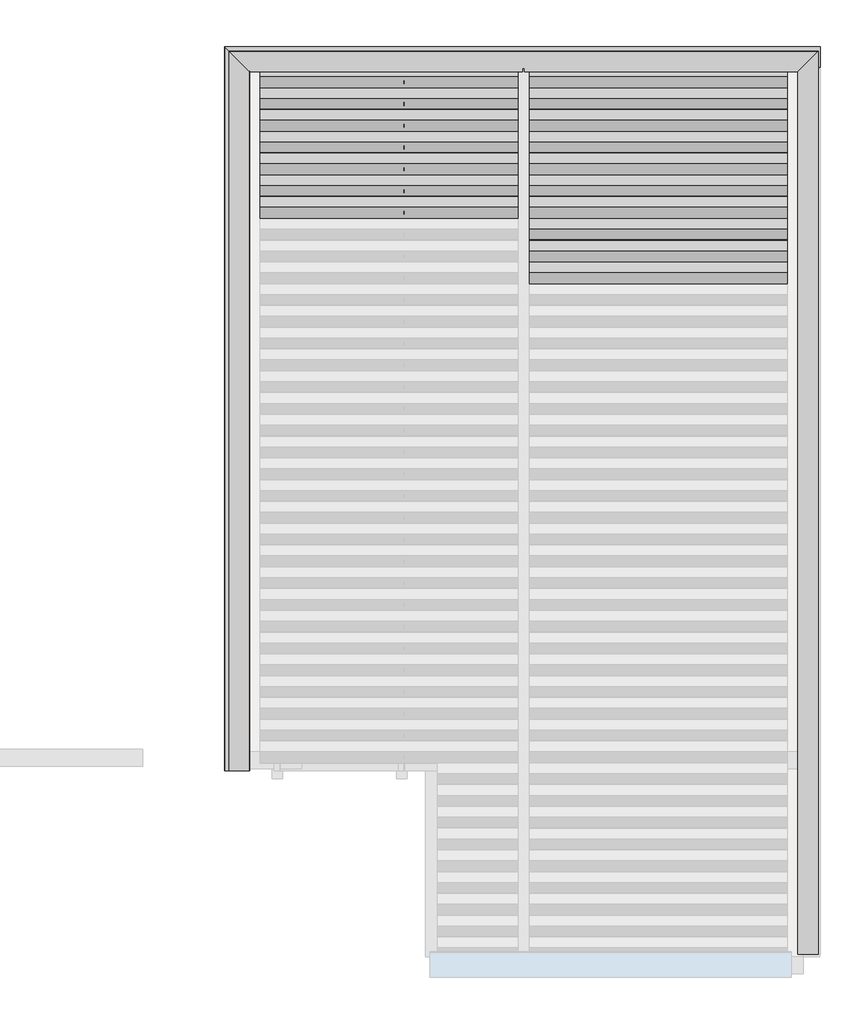
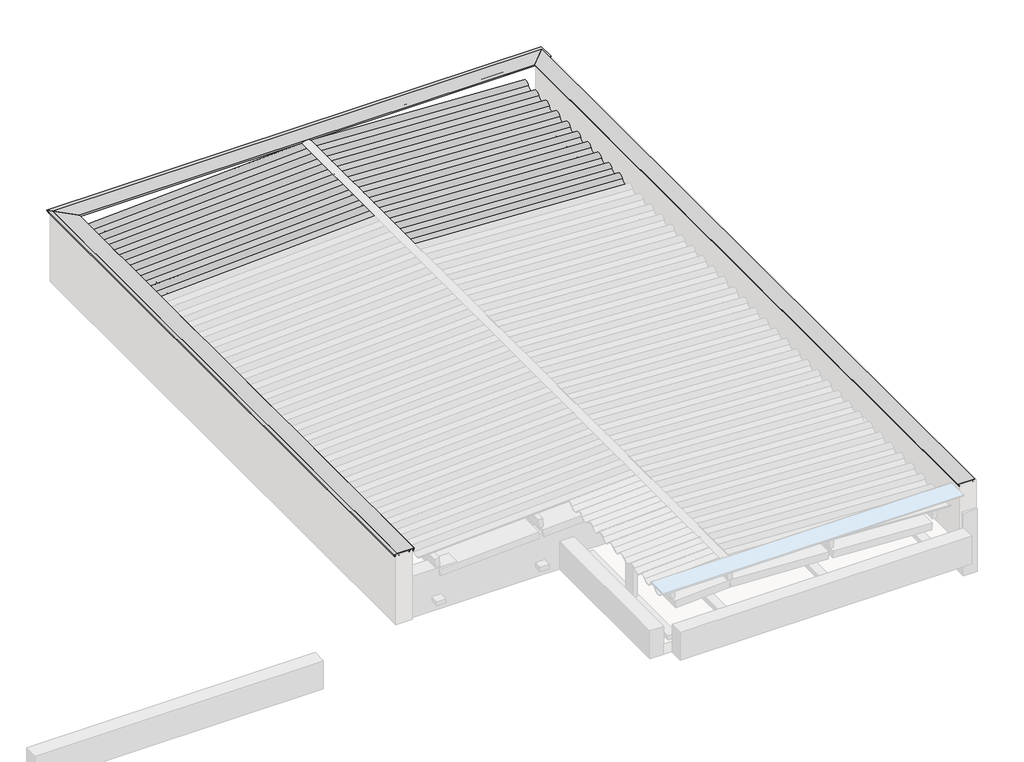
# One storey, part 4 of 4: 23 beams, 5 columns, 3 proxies.
# Revit data of these elements (continued)
# Elements 24, 26 (IfcBuildingElementProxy, ".CC_RUFO_PINGADEIRA_22 cm") (continued)
#   Materials on its faces: ".ALUMÍNIO COM PINTURA LÁTEX BRANCA"
# Element 25 (IfcBuildingElementProxy, ".CC_RUFO_PINGADEIRA_22 cm")
#   Uso = "TELHADOS RUFOS"
#   Nível de Ref. = "ESTAR/JANTAR/GALERIA"
#   Phase Created = CC_PE
#   Materials on its faces: ".ALUMÍNIO COM PINTURA LÁTEX BRANCA"
# Elements 27, 28, 29, 30, 31 (IfcColumn, "Madeira de lei-Coluna : Pontalete 6X16cm")
#   Comments = ""
#   Structural Material = .MADEIRAMENTO
#   Phase Created = CC_PE
#   Materials on its faces: ".MADEIRAMENTO"
# Materials
#   ".TELHA DE FIBROCIMENTO": class "CC_TELHADO", colour RGB 77 77 76, transparency 0, Description = "TELHA ONDULADA FIBROCIMENTO", Cost = 0
#   ".MADEIRAMENTO": class ".CC_MADEIRAS", colour RGB 212 179 113, transparency 0, Cost = 0
#   ".ALUMÍNIO COM PINTURA LÁTEX BRANCA": class "Generic", colour RGB 250 250 250, transparency 0, Cost = 0
